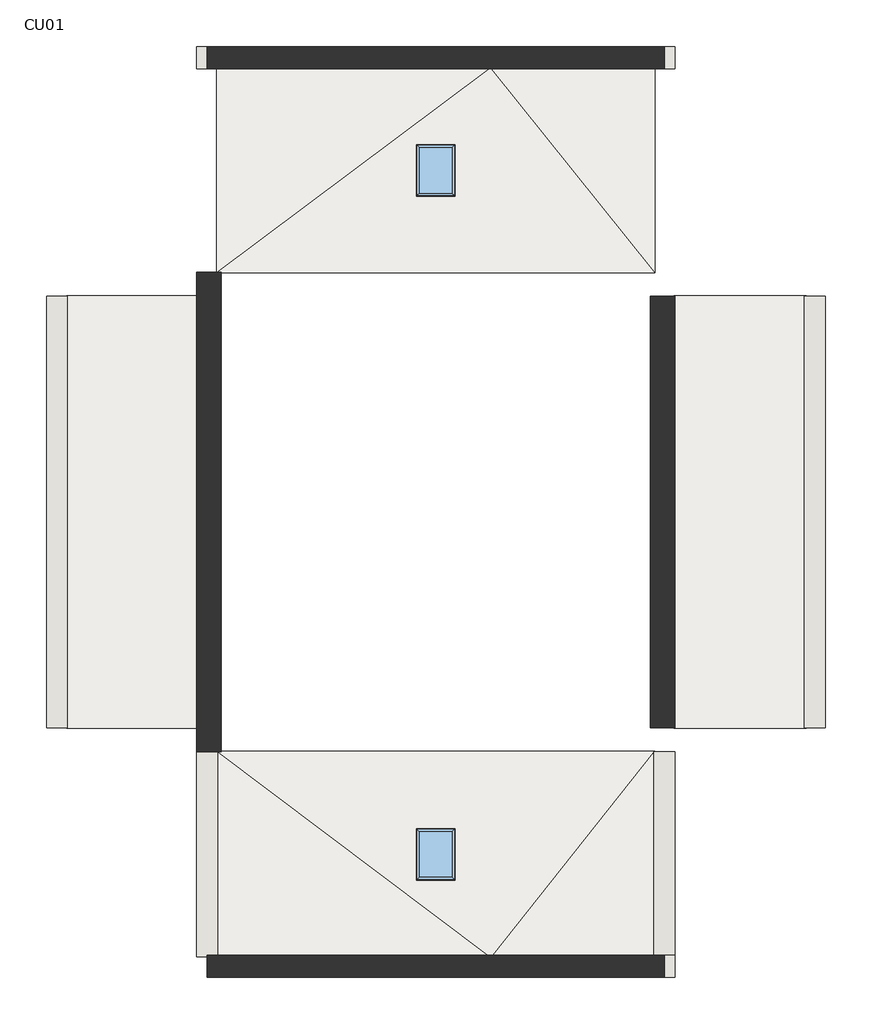
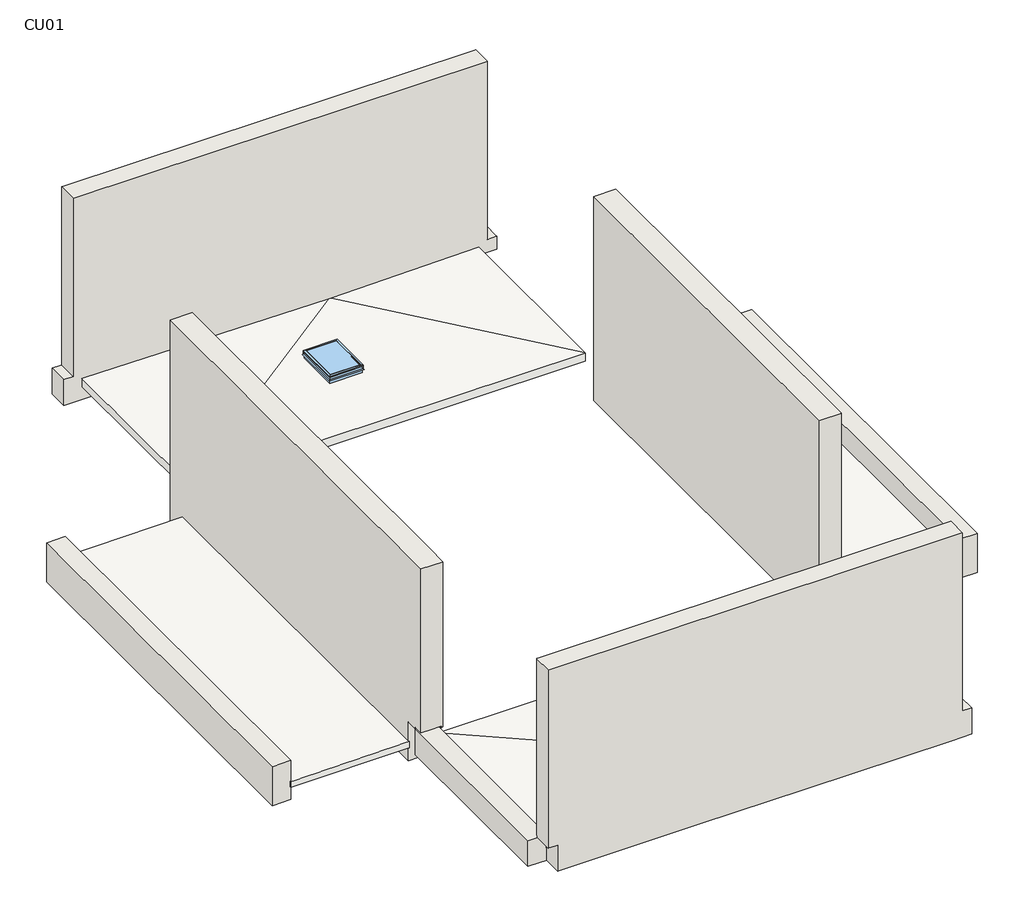
# One storey: 8 walls, 4 roofs, 2 windows.
"""IFC4 building model written with IfcOpenShell, lengths in millimetres."""

import ifcopenshell
import ifcopenshell.guid

model = None  # the IFC model being written
_history = None  # IfcOwnerHistory: only IFC2X3 demands one
_inside = {}  # id of a spatial element -> (the spatial element, [elements in it])
_under = {}  # id of a project, library or spatial element -> (it, [spatial elements below it])
_declared = {}  # id of a project -> (the project, [libraries it declares])
_typed = {}  # id of a type object -> (the type object, [elements of that type])
_made_of = {}  # id of a material, layer set ... -> (it, [elements and type objects made of it])


def new_model(schema):
    """Start an empty IFC model of exactly this schema.

    Asked for "IFC4X3", IfcOpenShell would pick the latest addendum, in which some entities
    have other attributes; the version numbers below select the first issue.
    IFC2X3 requires an IfcOwnerHistory on every rooted entity: one is made here for all.
    """
    global model, _history
    if schema == "IFC4X3":
        model = ifcopenshell.file(schema_version=(4, 3, 0, 0))
    else:
        model = ifcopenshell.file(schema=schema)
    _inside.clear()
    _under.clear()
    _declared.clear()
    _typed.clear()
    _made_of.clear()
    _history = None
    if model.schema == "IFC2X3":
        org = make("IfcOrganization", Name="unknown")
        user = make(
            "IfcPersonAndOrganization",
            ThePerson=make("IfcPerson", FamilyName="unknown"),
            TheOrganization=org,
        )
        app = make(
            "IfcApplication",
            ApplicationDeveloper=org,
            Version="unknown",
            ApplicationFullName="unknown",
            ApplicationIdentifier="unknown",
        )
        _history = make(
            "IfcOwnerHistory",
            OwningUser=user,
            OwningApplication=app,
            ChangeAction="ADDED",
            CreationDate=0,
        )
    return model


def make(cls, **values):
    """One entity of the class cls with the attributes given. An attribute that is None is left unset."""
    return model.create_entity(
        cls, **{name: value for name, value in values.items() if value is not None}
    )


def rooted(cls, **values):
    """An entity with a GlobalId (a new one), such as an element, a storey or a relation."""
    return make(cls, GlobalId=ifcopenshell.guid.new(), OwnerHistory=_history, **values)


def si_unit(unit_type, name, prefix=None):
    """IfcSIUnit, for example si_unit("LENGTHUNIT", "METRE", prefix="MILLI")."""
    return make("IfcSIUnit", UnitType=unit_type, Prefix=prefix, Name=name)


def assignment(units):
    """IfcUnitAssignment: the units of a project."""
    return None if units is None else make("IfcUnitAssignment", Units=units)


def point(xyz):
    """IfcCartesianPoint."""
    return None if xyz is None else make("IfcCartesianPoint", Coordinates=xyz)


def direction(xyz):
    """IfcDirection."""
    return None if xyz is None else make("IfcDirection", DirectionRatios=xyz)


def frame(location, z_axis=None, x_axis=None):
    """IfcAxis2Placement3D, a coordinate frame: its origin and axes. An axis left out is left unset."""
    return make(
        "IfcAxis2Placement3D",
        Location=point(location),
        Axis=direction(z_axis),
        RefDirection=direction(x_axis),
    )


def origin():
    """The frame at (0, 0, 0) with its axes left unset."""
    return frame((0.0, 0.0, 0.0))


def place(relative_to, where):
    """IfcLocalPlacement: puts the frame where relative to a parent placement (None: the world)."""
    return make(
        "IfcLocalPlacement", PlacementRelTo=relative_to, RelativePlacement=where
    )


def context(
    kind, dimensions, precision=None, world=None, true_north=None, identifier=None
):
    """IfcGeometricRepresentationContext, for example the 3D "Model" context."""
    return make(
        "IfcGeometricRepresentationContext",
        ContextIdentifier=identifier,
        ContextType=kind,
        CoordinateSpaceDimension=dimensions,
        Precision=precision,
        WorldCoordinateSystem=world,
        TrueNorth=true_north,
    )


def project(units=None, contexts=None):
    """IfcProject with its units and contexts."""
    return rooted(
        "IfcProject",
        Name="project",
        RepresentationContexts=contexts,
        UnitsInContext=assignment(units),
    )


def spatial(cls, under=None, at=None, **own):
    """A site, building, storey or space (cls), placed at a placement, below another one or the project."""
    s = rooted(cls, ObjectPlacement=at, **own)
    if under is not None:
        _under.setdefault(under.id(), (under, []))[1].append(s)
    return s


def polyline(points):
    """IfcPolyline through the points."""
    return make("IfcPolyline", Points=[point(p) for p in points])


def circle_curve(where, radius):
    """IfcCircle in the frame where."""
    return make("IfcCircle", Position=where, Radius=radius)


def outline(outer, holes=None, kind="AREA"):
    """IfcArbitraryClosedProfileDef: a profile drawn as a closed curve; with holes, ...WithVoids."""
    if holes is None:
        return make("IfcArbitraryClosedProfileDef", ProfileType=kind, OuterCurve=outer)
    return make(
        "IfcArbitraryProfileDefWithVoids",
        ProfileType=kind,
        OuterCurve=outer,
        InnerCurves=holes,
    )


def extrude(swept, where, along, depth):
    """IfcExtrudedAreaSolid: the profile swept, set in the frame where, extruded along a direction by depth."""
    return make(
        "IfcExtrudedAreaSolid",
        SweptArea=swept,
        Position=where,
        ExtrudedDirection=direction(along),
        Depth=depth,
    )


def faces_of(points, faces, orient=None, outer=None):
    """IfcFace entities. A face is a list of loops; a loop is a list of indices into points, from 0.

    orient and outer hold one flag for each loop. By default every Orientation is true, the
    first loop of a face is its IfcFaceOuterBound and the others are IfcFaceBound.
    """
    made = []
    for i, loops in enumerate(faces):
        bounds = []
        for j, loop in enumerate(loops):
            is_outer = j == 0 if outer is None else outer[i][j]
            bounds.append(
                make(
                    "IfcFaceOuterBound" if is_outer else "IfcFaceBound",
                    Bound=make("IfcPolyLoop", Polygon=[points[k] for k in loop]),
                    Orientation=True if orient is None else orient[i][j],
                )
            )
        made.append(make("IfcFace", Bounds=bounds))
    return made


def faceted_brep(points, faces, orient=None, outer=None, voids=None):
    """IfcFacetedBrep: a solid bounded by flat faces; with voids (closed shells), ...WithVoids."""
    shared = [point(p) for p in points]
    hull = make("IfcClosedShell", CfsFaces=faces_of(shared, faces, orient, outer))
    if voids is None:
        return make("IfcFacetedBrep", Outer=hull)
    return make(
        "IfcFacetedBrepWithVoids",
        Outer=hull,
        Voids=[
            make(cls, CfsFaces=faces_of(shared, fs, o, b)) for cls, fs, o, b in voids
        ],
    )


def shape(context_of_items, identifier, shape_type, items):
    """IfcShapeRepresentation: the items that make up one representation, for example the "Body"."""
    return make(
        "IfcShapeRepresentation",
        ContextOfItems=context_of_items,
        RepresentationIdentifier=identifier,
        RepresentationType=shape_type,
        Items=items,
    )


def source(mapping_origin, context_of_items, identifier, shape_type, items):
    """IfcRepresentationMap: a shape defined once, which mapped items show again and again."""
    return make(
        "IfcRepresentationMap",
        MappingOrigin=mapping_origin,
        MappedRepresentation=shape(context_of_items, identifier, shape_type, items),
    )


def transform(
    local_origin,
    x_axis=None,
    y_axis=None,
    z_axis=None,
    scale=None,
    scale2=None,
    scale3=None,
    uniform=True,
):
    """IfcCartesianTransformationOperator3D, or its non-uniform kind. x_axis, y_axis, z_axis: its Axis1, 2, 3."""
    if uniform:
        return make(
            "IfcCartesianTransformationOperator3D",
            Axis1=direction(x_axis),
            Axis2=direction(y_axis),
            LocalOrigin=point(local_origin),
            Scale=scale,
            Axis3=direction(z_axis),
        )
    return make(
        "IfcCartesianTransformationOperator3DnonUniform",
        Axis1=direction(x_axis),
        Axis2=direction(y_axis),
        LocalOrigin=point(local_origin),
        Scale=scale,
        Axis3=direction(z_axis),
        Scale2=scale2,
        Scale3=scale3,
    )


def mapped(mapping_source, mapping_target):
    """IfcMappedItem: shows the shape of a source again, moved by a transform."""
    return make(
        "IfcMappedItem", MappingSource=mapping_source, MappingTarget=mapping_target
    )


def made_of(thing, what):
    """Note that an element or type object is made of a material, layer set ...; save() writes the relation."""
    if what is not None:
        _made_of.setdefault(what.id(), (what, []))[1].append(thing)
    return thing


def element(
    cls,
    number,
    at=None,
    inside=None,
    cuts=None,
    type_object=None,
    material=None,
    context=None,
    identifier="Body",
    shape_type=None,
    held_by="IfcProductDefinitionShape",
    body=None,
    shapes=None,
    **own,
):
    """One element of the class cls, such as IfcWall. Its Tag is "e" and its number.

    at: its placement. inside: the storey or other place that contains it. cuts: it is an
    opening in that element (IfcRelVoidsElement). A single representation is given by context,
    identifier, shape_type and body (its items); several are given by shapes. held_by: the class
    of the entity that holds the representations. save() writes the other relations.
    """
    e = rooted(cls, Tag="e%d" % number, ObjectPlacement=at, **own)
    if body is not None:
        shapes = [shape(context, identifier, shape_type, body)]
    if shapes is not None:
        e.Representation = make(held_by, Representations=shapes)
    if inside is not None:
        _inside.setdefault(inside.id(), (inside, []))[1].append(e)
    if cuts is not None:
        rooted(
            "IfcRelVoidsElement", RelatingBuildingElement=cuts, RelatedOpeningElement=e
        )
    if type_object is not None:
        _typed.setdefault(type_object.id(), (type_object, []))[1].append(e)
    return made_of(e, material)


def aggregate(whole, parts):
    """IfcRelAggregates: a whole, such as a stair, and the parts it consists of."""
    return rooted("IfcRelAggregates", RelatingObject=whole, RelatedObjects=parts)


def save(model, path):
    """Write the relations noted so far, then the file.

    IfcRelAggregates (storeys below a building ...), IfcRelContainedInSpatialStructure (elements
    in a storey), IfcRelDefinesByType, IfcRelAssociatesMaterial and IfcRelDeclares: one each for
    every whole, place, type object, material and project.
    """
    for whole, parts in _under.values():
        aggregate(whole, parts)
    for where, things in _inside.values():
        rooted(
            "IfcRelContainedInSpatialStructure",
            RelatedElements=things,
            RelatingStructure=where,
        )
    for kind, things in _typed.values():
        rooted("IfcRelDefinesByType", RelatedObjects=things, RelatingType=kind)
    for what, things in _made_of.values():
        rooted("IfcRelAssociatesMaterial", RelatedObjects=things, RelatingMaterial=what)
    for by, libraries in _declared.values():
        rooted("IfcRelDeclares", RelatingContext=by, RelatedDefinitions=libraries)
    model.write(path)


def plane_surface(at):
    """IfcPlane: the flat surface through the origin of the frame at, square to its z axis."""
    return make("IfcPlane", Position=at)


def cylinder_surface(at, radius):
    """IfcCylindricalSurface: all points at the distance radius from the z axis of the frame at."""
    return make("IfcCylindricalSurface", Position=at, Radius=radius)


def advanced_brep(points, edges, surfaces, faces):
    """IfcAdvancedBrep: a solid bounded by faces that lie on surfaces and meet in shared edges.

    An edge is (start, end): straight between two places in points (the first is 0);
    or (start, end, curve); or (start, end, curve, False) where it runs against its curve.
    A face is (place in surfaces, loops), or (place, loops, False) where it looks against
    its surface's normal. A loop lists edges by number (the first is 1), with a minus sign
    where the edge is run from its end to its start. The first loop is the outer one.
    """
    corners = [point(p) for p in points]
    vertices = [make("IfcVertexPoint", VertexGeometry=c) for c in corners]
    made = []
    for start, end, *more in edges:
        made.append(
            make(
                "IfcEdgeCurve",
                EdgeStart=vertices[start],
                EdgeEnd=vertices[end],
                EdgeGeometry=more[0] if more else make("IfcPolyline", Points=[corners[start], corners[end]]),
                SameSense=more[1] if len(more) > 1 else True,
            )
        )
    hull = []
    for where, loops, *sense in faces:
        bounds = []
        for j, loop in enumerate(loops):
            ring = [make("IfcOrientedEdge", EdgeElement=made[abs(k) - 1], Orientation=k > 0) for k in loop]
            bounds.append(
                make(
                    "IfcFaceOuterBound" if j == 0 else "IfcFaceBound",
                    Bound=make("IfcEdgeLoop", EdgeList=ring),
                    Orientation=True,
                )
            )
        hull.append(make("IfcAdvancedFace", Bounds=bounds, FaceSurface=surfaces[where], SameSense=sense[0] if sense else True))
    return make("IfcAdvancedBrep", Outer=make("IfcClosedShell", CfsFaces=hull))


def claraboya_0711_x_0965mm_26b2130f(model_context):
    return source(origin(), model_context, "Body", "SolidModel", [
        faceted_brep([(254.440073, 370.1040988, 4001.2), (279.840073, 395.5040988, 4001.2), (279.840073, -569.4959012, 4001.2), (254.440073, -544.0959012, 4001.2), (254.440073, 370.1040988, 4026.6), (254.440073, -544.0959012, 4026.6), (292.540073, 408.2040988, 4026.6), (292.540073, -582.1959012, 4026.6), (292.540073, 408.2040988, 4001.2), (292.540073, -582.1959012, 4001.2), (292.540073, 408.2040988, 3950.4), (292.540073, -582.1959012, 3950.4), (307.1089145, 422.7729403, 3929.5935381), (307.1089145, -596.7647427, 3929.5935381), (301.907299, 417.5713248, 3925.9513277), (301.907299, -591.5631272, 3925.9513277), (286.190073, 401.8540988, 3948.3978527), (286.190073, -575.8459012, 3948.3978527), (286.190073, 401.8540988, 4001.2), (286.190073, -575.8459012, 4001.2), (-431.159927, -569.4959012, 4001.2), (-405.759927, -544.0959012, 4001.2), (-405.759927, -544.0959012, 4026.6), (-443.859927, -582.1959012, 4026.6), (-443.859927, -582.1959012, 4001.2), (-443.859927, -582.1959012, 3950.4), (-458.4287685, -596.7647427, 3929.5935381), (-453.227153, -591.5631272, 3925.9513277), (-437.509927, -575.8459012, 3948.3978527), (-437.509927, -575.8459012, 4001.2), (-431.159927, 395.5040988, 4001.2), (-405.759927, 370.1040988, 4001.2), (-405.759927, 370.1040988, 4026.6), (-443.859927, 408.2040988, 4026.6), (-443.859927, 408.2040988, 4001.2), (-443.859927, 408.2040988, 3950.4), (-458.4287685, 422.7729403, 3929.5935381), (-453.227153, 417.5713248, 3925.9513277), (-437.509927, 401.8540988, 3948.3978527), (-437.509927, 401.8540988, 4001.2)], [[[0, 1, 2, 3]], [[4, 0, 3, 5]], [[6, 4, 5, 7]], [[8, 6, 7, 9]], [[10, 8, 9, 11]], [[12, 10, 11, 13]], [[14, 12, 13, 15]], [[16, 14, 15, 17]], [[18, 16, 17, 19]], [[1, 18, 19, 2]], [[3, 2, 20, 21]], [[5, 3, 21, 22]], [[7, 5, 22, 23]], [[9, 7, 23, 24]], [[11, 9, 24, 25]], [[13, 11, 25, 26]], [[15, 13, 26, 27]], [[17, 15, 27, 28]], [[19, 17, 28, 29]], [[2, 19, 29, 20]], [[21, 20, 30, 31]], [[22, 21, 31, 32]], [[23, 22, 32, 33]], [[24, 23, 33, 34]], [[25, 24, 34, 35]], [[26, 25, 35, 36]], [[27, 26, 36, 37]], [[28, 27, 37, 38]], [[29, 28, 38, 39]], [[20, 29, 39, 30]], [[31, 30, 1, 0]], [[32, 31, 0, 4]], [[33, 32, 4, 6]], [[34, 33, 6, 8]], [[35, 34, 8, 10]], [[36, 35, 10, 12]], [[37, 36, 12, 14]], [[38, 37, 14, 16]], [[39, 38, 16, 18]], [[30, 39, 18, 1]]]),
        faceted_brep([(279.840073, -569.4959012, 4001.2), (279.840073, -569.4959012, 3848.8), (279.840073, 395.5040988, 3848.8), (279.840073, 395.5040988, 4001.2), (254.440073, -544.0959012, 4001.2), (254.440073, 370.1040988, 4001.2), (254.440073, -544.0959012, 3975.8), (254.440073, 370.1040988, 3975.8), (235.390073, -525.0459012, 3975.8), (235.390073, 351.0540988, 3975.8), (235.390073, -525.0459012, 3848.8), (235.390073, 351.0540988, 3848.8), (-431.159927, 395.5040988, 3848.8), (-431.159927, 395.5040988, 4001.2), (-405.759927, 370.1040988, 4001.2), (-405.759927, 370.1040988, 3975.8), (-386.709927, 351.0540988, 3975.8), (-386.709927, 351.0540988, 3848.8), (-431.159927, -569.4959012, 3848.8), (-431.159927, -569.4959012, 4001.2), (-405.759927, -544.0959012, 4001.2), (-405.759927, -544.0959012, 3975.8), (-386.709927, -525.0459012, 3975.8), (-386.709927, -525.0459012, 3848.8)], [[[0, 1, 2, 3]], [[4, 0, 3, 5]], [[6, 4, 5, 7]], [[8, 6, 7, 9]], [[10, 8, 9, 11]], [[1, 10, 11, 2]], [[3, 2, 12, 13]], [[5, 3, 13, 14]], [[7, 5, 14, 15]], [[9, 7, 15, 16]], [[11, 9, 16, 17]], [[2, 11, 17, 12]], [[13, 12, 18, 19]], [[14, 13, 19, 20]], [[15, 14, 20, 21]], [[16, 15, 21, 22]], [[17, 16, 22, 23]], [[12, 17, 23, 18]], [[19, 18, 1, 0]], [[20, 19, 0, 4]], [[21, 20, 4, 6]], [[22, 21, 6, 8]], [[23, 22, 8, 10]], [[18, 23, 10, 1]]]),
        extrude(outline(polyline([(254.440073, -544.0959012), (-405.759927, -544.0959012), (-405.759927, 370.1040988), (254.440073, 370.1040988), (254.440073, -544.0959012)])), frame((0.0, 0.0, 4020.25), z_axis=(0.0, 0.0, 1.0), x_axis=(1.0, 0.0, 0.0)), (0.0, 0.0, 1.0), 6.35),
    ])


def claraboya_0711_x_0965mm_17ef4467(model_context):
    return source(origin(), model_context, "Body", "SolidModel", [
        faceted_brep([(254.440073, -370.1040988, 4001.2), (254.440073, 544.0959012, 4001.2), (279.840073, 569.4959012, 4001.2), (279.840073, -395.5040988, 4001.2), (254.440073, -370.1040988, 4026.6), (254.440073, 544.0959012, 4026.6), (292.540073, -408.2040988, 4026.6), (292.540073, 582.1959012, 4026.6), (292.540073, -408.2040988, 4001.2), (292.540073, 582.1959012, 4001.2), (292.540073, -408.2040988, 3950.4), (292.540073, 582.1959012, 3950.4), (307.1089145, -422.7729403, 3929.5935381), (307.1089145, 596.7647427, 3929.5935381), (301.907299, -417.5713248, 3925.9513277), (301.907299, 591.5631272, 3925.9513277), (286.190073, -401.8540988, 3948.3978527), (286.190073, 575.8459012, 3948.3978527), (286.190073, -401.8540988, 4001.2), (286.190073, 575.8459012, 4001.2), (-405.759927, 544.0959012, 4001.2), (-431.159927, 569.4959012, 4001.2), (-405.759927, 544.0959012, 4026.6), (-443.859927, 582.1959012, 4026.6), (-443.859927, 582.1959012, 4001.2), (-443.859927, 582.1959012, 3950.4), (-458.4287685, 596.7647427, 3929.5935381), (-453.227153, 591.5631272, 3925.9513277), (-437.509927, 575.8459012, 3948.3978527), (-437.509927, 575.8459012, 4001.2), (-405.759927, -370.1040988, 4001.2), (-431.159927, -395.5040988, 4001.2), (-405.759927, -370.1040988, 4026.6), (-443.859927, -408.2040988, 4026.6), (-443.859927, -408.2040988, 4001.2), (-443.859927, -408.2040988, 3950.4), (-458.4287685, -422.7729403, 3929.5935381), (-453.227153, -417.5713248, 3925.9513277), (-437.509927, -401.8540988, 3948.3978527), (-437.509927, -401.8540988, 4001.2)], [[[0, 1, 2, 3]], [[4, 5, 1, 0]], [[6, 7, 5, 4]], [[8, 9, 7, 6]], [[10, 11, 9, 8]], [[12, 13, 11, 10]], [[14, 15, 13, 12]], [[16, 17, 15, 14]], [[18, 19, 17, 16]], [[3, 2, 19, 18]], [[1, 20, 21, 2]], [[5, 22, 20, 1]], [[7, 23, 22, 5]], [[9, 24, 23, 7]], [[11, 25, 24, 9]], [[13, 26, 25, 11]], [[15, 27, 26, 13]], [[17, 28, 27, 15]], [[19, 29, 28, 17]], [[2, 21, 29, 19]], [[20, 30, 31, 21]], [[22, 32, 30, 20]], [[23, 33, 32, 22]], [[24, 34, 33, 23]], [[25, 35, 34, 24]], [[26, 36, 35, 25]], [[27, 37, 36, 26]], [[28, 38, 37, 27]], [[29, 39, 38, 28]], [[21, 31, 39, 29]], [[30, 0, 3, 31]], [[32, 4, 0, 30]], [[33, 6, 4, 32]], [[34, 8, 6, 33]], [[35, 10, 8, 34]], [[36, 12, 10, 35]], [[37, 14, 12, 36]], [[38, 16, 14, 37]], [[39, 18, 16, 38]], [[31, 3, 18, 39]]]),
        faceted_brep([(279.840073, 569.4959012, 4001.2), (279.840073, -395.5040988, 4001.2), (279.840073, -395.5040988, 3848.8), (279.840073, 569.4959012, 3848.8), (254.440073, 544.0959012, 4001.2), (254.440073, -370.1040988, 4001.2), (254.440073, 544.0959012, 3975.8), (254.440073, -370.1040988, 3975.8), (235.390073, 525.0459012, 3975.8), (235.390073, -351.0540988, 3975.8), (235.390073, 525.0459012, 3848.8), (235.390073, -351.0540988, 3848.8), (-431.159927, -395.5040988, 4001.2), (-431.159927, -395.5040988, 3848.8), (-405.759927, -370.1040988, 4001.2), (-405.759927, -370.1040988, 3975.8), (-386.709927, -351.0540988, 3975.8), (-386.709927, -351.0540988, 3848.8), (-431.159927, 569.4959012, 4001.2), (-431.159927, 569.4959012, 3848.8), (-405.759927, 544.0959012, 4001.2), (-405.759927, 544.0959012, 3975.8), (-386.709927, 525.0459012, 3975.8), (-386.709927, 525.0459012, 3848.8)], [[[0, 1, 2, 3]], [[4, 5, 1, 0]], [[6, 7, 5, 4]], [[8, 9, 7, 6]], [[10, 11, 9, 8]], [[3, 2, 11, 10]], [[1, 12, 13, 2]], [[5, 14, 12, 1]], [[7, 15, 14, 5]], [[9, 16, 15, 7]], [[11, 17, 16, 9]], [[2, 13, 17, 11]], [[12, 18, 19, 13]], [[14, 20, 18, 12]], [[15, 21, 20, 14]], [[16, 22, 21, 15]], [[17, 23, 22, 16]], [[13, 19, 23, 17]], [[18, 0, 3, 19]], [[20, 4, 0, 18]], [[21, 6, 4, 20]], [[22, 8, 6, 21]], [[23, 10, 8, 22]], [[19, 3, 10, 23]]]),
        extrude(outline(polyline([(254.440073, 544.0959012), (254.440073, -370.1040988), (-405.759927, -370.1040988), (-405.759927, 544.0959012), (254.440073, 544.0959012)])), frame((0.0, 0.0, 4020.25), z_axis=(0.0, 0.0, 1.0), x_axis=(1.0, 0.0, 0.0)), (0.0, 0.0, 1.0), 6.35),
    ])


model = new_model("IFC4")

# Units and contexts
model_context = context("Model", 3, world=origin())
ifc_project = project(units=[si_unit("LENGTHUNIT", "METRE", prefix="MILLI")], contexts=[model_context])

# Site, building, storey
site = spatial("IfcSite", under=ifc_project)
building = spatial("IfcBuilding", under=site)
storey = spatial("IfcBuildingStorey", under=building, Name="CU01", Elevation=2430.0)

# Roofs
placement = place(None, origin())
element("IfcRoof", 1, ObjectType="ACAB CUB GRAVA INF-A_PABLO", at=placement, inside=storey, context=model_context, shape_type="Brep", body=[
    faceted_brep([(-12165.0, -4267.5, 2730.0), (-12165.0, -4252.5, 2730.0), (-12165.0, -232.5, 2730.0), (-12165.0, -217.5, 2730.0), (-12165.0, -217.5, 2921.2), (-12165.0, -232.5, 2921.2), (-12165.0, -4252.5, 2921.2), (-12165.0, -4267.5, 2921.2), (-12235.0, -217.5, 2730.0), (-20835.0, -217.5, 2730.0), (-20835.0, -217.5, 2921.2), (-15415.0, -217.5, 2871.2), (-16188.95, -1804.45, 2890.7919753), (-16188.95, -1804.45, 2730.0), (-16188.95, -2680.55, 2730.0), (-16188.95, -2680.55, 2901.6080247), (-16811.05, -2680.55, 2730.0), (-16811.05, -2680.55, 2901.6080247), (-16811.05, -1804.45, 2730.0), (-16811.05, -1804.45, 2890.7919753), (-20750.0, -4267.5, 2730.0), (-20835.0, -4267.5, 2730.0), (-20835.0, -4252.5, 2730.0), (-20835.0, -232.5, 2730.0), (-20835.0, -4267.5, 2921.2), (-20835.0, -4252.5, 2921.2), (-20835.0, -232.5, 2921.2), (-20750.0, -4267.5, 2921.2), (-12177.037037, -4252.5, 2921.0148148), (-12180.0, -4248.8076923, 2920.9692308), (-15402.962963, -232.5, 2871.3851852), (-15435.0740741, -232.5, 2871.3851852)], [[[0, 1, 2, 3, 4, 5, 6, 7]], [[3, 8, 9, 10, 11, 4]], [[12, 13, 14, 15]], [[15, 14, 16, 17]], [[17, 16, 18, 19]], [[13, 12, 19, 18]], [[3, 2, 1, 0, 20, 21, 22, 23, 9, 8], [14, 13, 18, 16]], [[9, 23, 22, 21, 24, 25, 26, 10]], [[0, 7, 27, 24, 21, 20]], [[24, 27, 7, 28, 29, 30, 11, 31], [12, 15, 17, 19]], [[7, 6, 5, 4, 11, 30, 29, 28]], [[10, 26, 25, 24, 31, 11]]]),
])
element("IfcRoof", 2, ObjectType="ACAB CUB GRAVA INF-B_PABLO", at=placement, inside=storey, context=model_context, shape_type="Brep", body=[
    faceted_brep([(-23810.0, -4717.5, 2430.0), (-21230.0, -4717.5, 2430.0), (-21215.0, -4717.5, 2430.0), (-21215.0, -13267.5, 2430.0), (-21215.0, -13282.5, 2430.0), (-21230.0, -13282.5, 2430.0), (-23810.0, -13282.5, 2430.0), (-23810.0, -13267.5, 2430.0), (-23810.0, -4732.5, 2430.0), (-21215.0, -4717.5, 2581.2), (-23810.0, -4717.5, 2551.2), (-21230.0, -4717.5, 2581.0265896), (-23810.0, -13282.5, 2551.2), (-23810.0, -13267.5, 2551.2), (-23810.0, -9000.0, 2551.2), (-23810.0, -4732.5, 2551.2), (-21215.0, -13282.5, 2581.2), (-21215.0, -13267.5, 2581.2)], [[[0, 1, 2, 3, 4, 5, 6, 7, 8]], [[9, 2, 1, 0, 10, 11]], [[10, 0, 8, 7, 6, 12, 13, 14, 15]], [[12, 6, 5, 4, 16]], [[10, 15, 14, 13, 12, 16, 17, 9, 11]], [[16, 4, 3, 2, 9, 17]]]),
])
element("IfcRoof", 3, ObjectType="ACAB CUB GRAVA INF-A_PABLO", at=placement, inside=storey, context=model_context, shape_type="Brep", body=[
    faceted_brep([(-12165.0, -17812.5, 2730.0), (-12165.0, -17767.5, 2730.0), (-12165.0, -13747.5, 2730.0), (-12165.0, -13732.5, 2730.0), (-12165.0, -13732.5, 2921.2), (-12165.0, -13747.5, 2921.2), (-12165.0, -17767.5, 2921.2), (-12165.0, -17812.5, 2921.2), (-15405.0, -17812.5, 2871.2), (-20820.0, -17812.5, 2921.0618785), (-20835.0, -17812.5, 2921.2), (-20835.0, -17812.5, 2730.0), (-20820.0, -17812.5, 2730.0), (-16188.95, -16210.55, 2730.0), (-16188.95, -16210.55, 2890.8317402), (-16188.95, -15334.45, 2901.5682598), (-16188.95, -15334.45, 2730.0), (-16811.05, -15334.45, 2901.5682598), (-16811.05, -15334.45, 2730.0), (-16811.05, -16210.55, 2890.8317402), (-16811.05, -16210.55, 2730.0), (-20835.0, -17797.5, 2730.0), (-20835.0, -13732.5, 2730.0), (-20820.0, -13732.5, 2730.0), (-20750.0, -13732.5, 2730.0), (-20835.0, -17797.5, 2921.2), (-20835.0, -13732.5, 2921.2), (-20820.0, -13732.5, 2921.2), (-20750.0, -13732.5, 2921.2), (-12176.9117647, -13747.5, 2921.0161765), (-12180.0, -13751.3888889, 2920.9685185), (-15369.2647059, -17767.5, 2871.7514706), (-20820.0, -13743.7707182, 2921.0618785), (-15464.8897059, -17767.5, 2871.7514706)], [[[0, 1, 2, 3, 4, 5, 6, 7]], [[0, 7, 8, 9, 10, 11, 12]], [[13, 14, 15, 16]], [[16, 15, 17, 18]], [[18, 17, 19, 20]], [[14, 13, 20, 19]], [[3, 2, 1, 0, 12, 11, 21, 22, 23, 24], [13, 16, 18, 20]], [[22, 21, 11, 10, 25, 26]], [[4, 3, 24, 23, 22, 26, 27, 28]], [[7, 6, 5, 4, 29, 30, 31, 8]], [[4, 28, 27, 26, 32, 33, 8, 31, 30, 29], [15, 14, 19, 17]], [[26, 25, 10, 9, 8, 33, 32]]]),
])
element("IfcRoof", 4, ObjectType="ACAB CUB GRAVA INF-B_PABLO", at=placement, inside=storey, context=model_context, shape_type="Brep", body=[
    faceted_brep([(-11785.0, -4717.5, 2430.0), (-9165.0, -4717.5, 2430.0), (-9165.0, -4732.5, 2430.0), (-9165.0, -13267.5, 2430.0), (-9165.0, -13282.5, 2430.0), (-11785.0, -13282.5, 2430.0), (-11785.0, -13267.5, 2430.0), (-11785.0, -4732.5, 2430.0), (-9165.0, -4717.5, 2551.2), (-11785.0, -4717.5, 2581.2), (-9165.0, -13282.5, 2551.2), (-9165.0, -4732.5, 2551.2), (-9165.0, -9000.0, 2551.2), (-9165.0, -13267.5, 2551.2), (-11785.0, -13282.5, 2581.2), (-11785.0, -4732.5, 2581.2), (-11785.0, -13267.5, 2581.2)], [[[0, 1, 2, 3, 4, 5, 6, 7]], [[8, 1, 0, 9]], [[10, 4, 3, 2, 1, 8, 11, 12, 13]], [[14, 5, 4, 10]], [[12, 11, 8, 9, 15, 16, 14, 10, 13]], [[9, 0, 7, 6, 5, 14, 16, 15]]]),
])

# Walls
element("IfcWall", 5, ObjectType="MURO TIPO 1_EXTERIOR_PETO_PABLO", at=placement, inside=storey, context=model_context, shape_type="Brep", body=[
    faceted_brep([(-23795.0, -13267.5, 2130.0), (-23795.0, -4732.5, 2130.0), (-23795.0, -4732.5, 2430.0), (-23795.0, -13267.5, 2430.0), (-23795.0, -4732.5, 3030.0), (-23795.0, -13267.5, 3030.0), (-23795.0, -13267.5, 2551.3734104), (-23795.0, -4732.5, 2551.3734104), (-24205.0, -4732.5, 2130.0), (-24205.0, -13267.5, 2130.0), (-24205.0, -13267.5, 3030.0), (-24205.0, -4732.5, 3030.0), (-23810.0, -13267.5, 2430.0), (-23810.0, -13267.5, 2551.2), (-23810.0, -4732.5, 2551.2), (-23810.0, -4732.5, 2430.0), (-23810.0, -9000.0, 2551.2)], [[[0, 1, 2, 3]], [[4, 5, 6, 7]], [[8, 9, 10, 11]], [[1, 0, 9, 8]], [[5, 4, 11, 10]], [[5, 10, 9, 0, 3, 12, 13, 6]], [[1, 8, 11, 4, 7, 14, 15, 2]], [[15, 12, 3, 2]], [[12, 15, 14, 16, 13]], [[13, 16, 14, 7, 6]]]),
])
element("IfcWall", 6, ObjectType="MURO TIPO 1_EXTERIOR_PETO_PABLO", at=placement, inside=storey, context=model_context, shape_type="Brep", body=[
    faceted_brep([(-8795.0, -13267.5, 2130.0), (-8795.0, -4732.5, 2130.0), (-8795.0, -4732.5, 3030.0), (-8795.0, -13267.5, 3030.0), (-9205.0, -4732.5, 2130.0), (-9205.0, -13267.5, 2130.0), (-9205.0, -13267.5, 2430.0), (-9205.0, -4732.5, 2430.0), (-9205.0, -13267.5, 3030.0), (-9205.0, -4732.5, 3030.0), (-9205.0, -4732.5, 2551.6580153), (-9205.0, -13267.5, 2551.6580153), (-9165.0, -13267.5, 2551.2), (-9165.0, -13267.5, 2430.0), (-9165.0, -4732.5, 2430.0), (-9165.0, -4732.5, 2551.2), (-9165.0, -9000.0, 2551.2)], [[[0, 1, 2, 3]], [[4, 5, 6, 7]], [[8, 9, 10, 11]], [[1, 0, 5, 4]], [[3, 2, 9, 8]], [[0, 3, 8, 11, 12, 13, 6, 5]], [[2, 1, 4, 7, 14, 15, 10, 9]], [[13, 14, 7, 6]], [[14, 13, 12, 16, 15]], [[16, 12, 11, 10, 15]]]),
])
element("IfcWall", 7, ObjectType="MURO TIPO 1_EXTERIOR_PETO-CUB_PABLO", at=placement, inside=storey, context=model_context, shape_type="Brep", body=[
    faceted_brep([(-21230.0, -232.5, 2430.0), (-12235.0, -232.5, 2430.0), (-12235.0, -232.5, 2730.0), (-20835.0, -232.5, 2730.0), (-20835.0, -232.5, 2921.2), (-15435.0740741, -232.5, 2871.3851852), (-15402.962963, -232.5, 2871.3851852), (-12180.0, -232.5, 2920.9692308), (-12165.0, -232.5, 2921.2), (-12165.0, -232.5, 2730.0), (-11770.0, -232.5, 2730.0), (-11770.0, -232.5, 3030.0), (-11975.0, -232.5, 3030.0), (-11975.0, -232.5, 7150.0), (-12002.5, -232.5, 7150.0), (-21010.0, -232.5, 7150.0), (-21025.0, -232.5, 7150.0), (-21025.0, -232.5, 3030.0), (-21230.0, -232.5, 3030.0), (-21230.0, -232.5, 2730.0), (-12235.0, 207.5, 2430.0), (-17710.0, 207.5, 2430.0), (-21230.0, 207.5, 2430.0), (-21230.0, 207.5, 3030.0), (-21025.0, 207.5, 3030.0), (-21025.0, 207.5, 7150.0), (-21010.0, 207.5, 7150.0), (-12002.5, 207.5, 7150.0), (-11975.0, 207.5, 7150.0), (-11975.0, 207.5, 3030.0), (-11770.0, 207.5, 3030.0), (-11770.0, 207.5, 2730.0), (-12235.0, 207.5, 2730.0), (-12165.0, -217.5, 2730.0), (-12235.0, -217.5, 2730.0), (-12165.0, -217.5, 2921.2), (-15415.0, -217.5, 2871.2), (-20835.0, -217.5, 2921.2), (-20835.0, -217.5, 2730.0), (-21230.0, 192.5, 3030.0), (-21230.0, -217.5, 3030.0), (-11770.0, -217.5, 3030.0), (-11770.0, 192.5, 3030.0)], [[[0, 1, 2, 3, 4, 5, 6, 7, 8, 9, 10, 11, 12, 13, 14, 15, 16, 17, 18, 19]], [[20, 21, 22, 23, 24, 25, 26, 27, 28, 29, 30, 31, 32]], [[1, 0, 22, 21, 20]], [[16, 15, 14, 13, 28, 27, 26, 25]], [[32, 31, 10, 9, 33, 34]], [[2, 1, 20, 32, 34]], [[33, 35, 36, 37, 38, 34]], [[35, 33, 9, 8]], [[34, 38, 3, 2]], [[38, 37, 4, 3]], [[16, 25, 24, 17]], [[17, 24, 23, 39, 40, 18]], [[22, 0, 19, 18, 40, 39, 23]], [[36, 35, 8, 7, 6]], [[37, 36, 5, 4]], [[36, 6, 5]], [[28, 13, 12, 29]], [[29, 12, 11, 41, 42, 30]], [[11, 10, 31, 30, 42, 41]]]),
])
element("IfcWall", 8, ObjectType="MURO TIPO 3B_ESTAR-EXT_YESO-CEMENTO_PABLO", at=placement, inside=storey, context=model_context, shape_type="Brep", body=[
    faceted_brep([(-12250.0, -4732.5, 2130.0), (-12250.0, -13267.5, 2130.0), (-12250.0, -13267.5, 6850.0), (-12250.0, -4732.5, 6850.0), (-11770.0, -13267.5, 2130.0), (-11770.0, -4732.5, 2130.0), (-11770.0, -4732.5, 2430.0), (-11770.0, -13267.5, 2430.0), (-11770.0, -4732.5, 6850.0), (-11770.0, -13267.5, 6850.0), (-11770.0, -13267.5, 2581.0282443), (-11770.0, -4732.5, 2581.0282443), (-11785.0, -13267.5, 2130.0), (-11785.0, -13267.5, 6850.0), (-11785.0, -4732.5, 2430.0), (-11785.0, -13267.5, 2430.0), (-11785.0, -13267.5, 2581.2), (-11785.0, -4732.5, 2581.2)], [[[0, 1, 2, 3]], [[4, 5, 6, 7]], [[8, 9, 10, 11]], [[1, 0, 5, 4, 12]], [[3, 2, 13, 9, 8]], [[14, 15, 7, 6]], [[16, 17, 11, 10]], [[15, 14, 17, 16]], [[1, 12, 4, 7, 15, 16, 10, 9, 13, 2]], [[5, 0, 3, 8, 11, 17, 14, 6]]]),
])
element("IfcWall", 9, ObjectType="MURO TIPO 1_EXTERIOR_PETO_PABLO", at=placement, inside=storey, context=model_context, shape_type="Brep", body=[
    faceted_brep([(-11770.0, -17767.5, 2430.0), (-11770.0, -13747.5, 2430.0), (-11770.0, -13747.5, 3030.0), (-11770.0, -17767.5, 3030.0), (-12180.0, -13747.5, 2430.0), (-12180.0, -17767.5, 2430.0), (-12180.0, -17767.5, 2730.0), (-12180.0, -13747.5, 2730.0), (-12180.0, -17767.5, 3030.0), (-12180.0, -13747.5, 3030.0), (-12180.0, -13747.5, 2921.0161765), (-12180.0, -13751.3888889, 2920.9685185), (-12180.0, -17767.5, 2920.9685185), (-11975.0, -17767.5, 3030.0), (-12165.0, -13747.5, 2921.2), (-12165.0, -13747.5, 2730.0), (-12165.0, -17767.5, 2730.0), (-12165.0, -17767.5, 2921.2), (-12176.9117647, -13747.5, 2921.0161765)], [[[0, 1, 2, 3]], [[4, 5, 6, 7]], [[8, 9, 10, 11, 12]], [[1, 0, 5, 4]], [[3, 2, 9, 8, 13]], [[14, 15, 16, 17]], [[7, 6, 16, 15]], [[11, 18, 14, 17, 12]], [[18, 11, 10]], [[2, 1, 4, 7, 15, 14, 18, 10, 9]], [[0, 3, 13, 8, 12, 17, 16, 6, 5]]]),
])
element("IfcWall", 10, ObjectType="MURO TIPO 1_EXTERIOR_PETO_PABLO", at=placement, inside=storey, context=model_context, shape_type="Brep", body=[
    faceted_brep([(-20820.0, -17797.5, 2430.0), (-20820.0, -17767.5, 2430.0), (-20820.0, -13537.5, 2430.0), (-20820.0, -13537.5, 3030.0), (-20820.0, -17767.5, 3030.0), (-20820.0, -17797.5, 3030.0), (-20820.0, -17797.5, 2921.0618785), (-20820.0, -17767.5, 2921.0618785), (-20820.0, -13743.7707182, 2921.0618785), (-20820.0, -13732.5, 2921.2), (-20820.0, -13732.5, 2730.0), (-20820.0, -17767.5, 2730.0), (-20820.0, -17797.5, 2730.0), (-21230.0, -13537.5, 2430.0), (-21230.0, -17797.5, 2430.0), (-21230.0, -17797.5, 3030.0), (-21230.0, -13537.5, 3030.0), (-21010.0, -17797.5, 3030.0), (-20835.0, -13732.5, 2730.0), (-20835.0, -17797.5, 2730.0), (-20835.0, -13732.5, 2921.2), (-20835.0, -17797.5, 2921.2)], [[[0, 1, 2, 3, 4, 5, 6, 7, 8, 9, 10, 11, 12]], [[13, 14, 15, 16]], [[2, 1, 0, 14, 13]], [[5, 4, 3, 16, 15, 17]], [[10, 18, 19, 12, 11]], [[18, 20, 21, 19]], [[20, 9, 8]], [[20, 8, 7, 6, 21]], [[3, 2, 13, 16]], [[20, 18, 10, 9]], [[5, 17, 15, 14, 0, 12, 19, 21, 6]]]),
])
element("IfcWall", 11, ObjectType="MURO TIPO 3B_ESTAR-EXT_YESO-CEMENTO_PABLO", at=placement, inside=storey, context=model_context, shape_type="AdvancedBrep", body=[
    advanced_brep(
    [(-21230.0, -4252.5, 2130.0), (-21230.0, -13267.5, 2130.0), (-21230.0, -13267.5, 2430.0), (-21230.0, -13267.5, 3030.0), (-21230.0, -13537.5, 3030.0), (-21230.0, -13537.5, 3060.7854779), (-21230.0, -13747.5, 3060.7854779), (-21230.0, -13747.5, 6850.0), (-21230.0, -4252.5, 6850.0), (-20750.0, -13267.5, 2130.0), (-20750.0, -4732.5, 2130.0), (-20750.0, -4252.5, 2130.0), (-20750.0, -4252.5, 2730.0), (-20750.0, -4252.5, 2921.0148148), (-20750.0, -4252.5, 6850.0), (-20750.0, -4732.5, 6850.0), (-20750.0, -13267.5, 6850.0), (-20750.0, -13747.5, 6850.0), (-20750.0, -13747.5, 3030.0), (-20750.0, -13537.5, 3030.0), (-20750.0, -13267.5, 3030.0), (-20750.0, -13267.5, 2430.0), (-20790.0, -13267.5, 2130.0), (-20775.0, -13537.5, 3030.0), (-20775.0, -13537.5, 3060.0), (-21025.0, -13537.5, 3064.3637662), (-20820.0, -13537.5, 3030.0), (-20804.8467624, -13537.5, 3030.0), (-20789.8467624, -13537.5, 3030.0), (-20775.0, -13747.5, 3030.0), (-20775.0, -13747.5, 3060.0), (-20804.8467624, -13747.5, 3030.0), (-20789.8467624, -13747.5, 3030.0), (-21025.0, -13747.5, 3064.3637662)],
    [
        (0, 1),
        (1, 2),
        (2, 3),
        (3, 4),
        (4, 5),
        (5, 6),
        (6, 7),
        (7, 8),
        (8, 0),
        (9, 10),
        (10, 11),
        (11, 12),
        (12, 13),
        (13, 14),
        (14, 15),
        (15, 16),
        (16, 17),
        (17, 18),
        (18, 19),
        (19, 20),
        (20, 21),
        (21, 9),
        (0, 11),
        (9, 22),
        (22, 1),
        (7, 17),
        (14, 8),
        (23, 24),
        (24, 25),
        (25, 5),
        (4, 26),
        (26, 27),
        (27, 28, circle_curve(frame((-20797.3467624, -13537.5, 3030.0), z_axis=(0.0, 1.0, 0.0), x_axis=(-1.0, 0.0, 0.0)), 7.5)),
        (28, 23),
        (23, 29),
        (29, 30),
        (30, 24),
        (27, 31),
        (31, 32, circle_curve(frame((-20797.3467624, -13747.5, 3030.0), z_axis=(0.0, 1.0, 0.0), x_axis=(-1.0, 0.0, 0.0)), 7.5)),
        (32, 28),
        (25, 33),
        (33, 6),
        (30, 33),
        (20, 3),
        (29, 18),
        (31, 32),
    ],
    [
        plane_surface(frame((-21230.0, -4500.0, 2130.0), z_axis=(-1.0, 0.0, 0.0), x_axis=(0.0, -1.0, 0.0))),
        plane_surface(frame((-20750.0, -4500.0, 2130.0), z_axis=(1.0, 0.0, 0.0), x_axis=(0.0, 1.0, 0.0))),
        plane_surface(frame((-21230.0, -4492.5, 2130.0), z_axis=(0.0, 0.0, -1.0), x_axis=(1.0, 0.0, 0.0))),
        plane_surface(frame((-21230.0, -13507.5, 6850.0), z_axis=(0.0, 0.0, 1.0), x_axis=(1.0, 0.0, 0.0))),
        plane_surface(frame((-21010.0, -4252.5, 2130.0), z_axis=(0.0, 1.0, 0.0), x_axis=(-1.0, 0.0, 0.0))),
        plane_surface(frame((-21685.9879384, -13537.5, 3030.0), z_axis=(0.0, -1.0, 0.0), x_axis=(0.0, 0.0, 1.0))),
        plane_surface(frame((-20775.0, -17797.5, 3030.0), z_axis=(-1.0, 0.0, 0.0), x_axis=(0.0, 1.0, 0.0))),
        cylinder_surface(frame((-20797.3467624, -17797.5, 3030.0), z_axis=(0.0, 1.0, 0.0), x_axis=(-1.0, 0.0, 0.0)), 7.5),
        plane_surface(frame((-21025.0, -17797.5, 3064.3637662), z_axis=(0.017452406437287852, 0.0, -0.9998476951563912), x_axis=(0.0, 1.0, 0.0))),
        plane_surface(frame((-20775.0, -17797.5, 3060.0), z_axis=(-0.01745240643728998, 0.0, -0.9998476951563912), x_axis=(0.0, 1.0, 0.0))),
        plane_surface(frame((-19420.0, -13267.5, -135.0), z_axis=(0.0, -1.0, 0.0), x_axis=(-1.0, 0.0, 0.0))),
        plane_surface(frame((-11785.0, -13747.5, 2130.0), z_axis=(0.0, -1.0, 0.0), x_axis=(1.0, 0.0, 0.0))),
        plane_surface(frame((-21230.0, -13507.5, 3030.0), z_axis=(0.0, 0.0, -1.0), x_axis=(1.0, 0.0, 0.0))),
    ],
    [
        (0, [[1, 2, 3, 4, 5, 6, 7, 8, 9]]),
        (1, [[10, 11, 12, 13, 14, 15, 16, 17, 18, 19, 20, 21, 22]]),
        (2, [[-1, 23, -11, -10, 24, 25]]),
        (3, [[-8, 26, -17, -16, -15, 27]]),
        (4, [[-9, -27, -14, -13, -12, -23]]),
        (5, [[28, 29, 30, -5, 31, 32, 33, 34]]),
        (6, [[-28, 35, 36, 37]]),
        (7, [[-33, 38, 39, 40]]),
        (8, [[-30, 41, 42, -6]]),
        (9, [[-29, -37, 43, -41]]),
        (10, [[-3, -2, -25, -24, -22, -21, 44]]),
        (11, [[-18, -26, -7, -42, -43, -36, 45]]),
        (11, [[46, -39]]),
        (12, [[-20, -19, -45, -35, -34, -40, -46, -38, -32, -31, -4, -44]]),
    ],
),
])
element("IfcWall", 12, ObjectType="MURO TIPO 1_EXTERIOR_PETO-CUB_PABLO", at=placement, inside=storey, context=model_context, shape_type="AdvancedBrep", body=[
    advanced_brep(
    [(-20820.0, -18207.5, 2430.0), (-20790.0, -18207.5, 2430.0), (-17710.0, -18207.5, 2430.0), (-15417.5, -18207.5, 2430.0), (-12210.0, -18207.5, 2430.0), (-11770.0, -18207.5, 2430.0), (-11770.0, -18207.5, 3030.0), (-11975.0, -18207.5, 3030.0), (-11975.0, -18207.5, 7150.0), (-11990.0, -18207.5, 7150.0), (-21010.0, -18207.5, 7150.0), (-21025.0, -18207.5, 7150.0), (-21025.0, -18207.5, 3030.0), (-21010.0, -18207.5, 3030.0), (-20820.0, -18207.5, 3030.0), (-11770.0, -17767.5, 2430.0), (-12180.0, -17767.5, 2430.0), (-20820.0, -17767.5, 2430.0), (-20820.0, -17767.5, 2730.0), (-12180.0, -17767.5, 2730.0), (-12165.0, -17767.5, 2730.0), (-12165.0, -17767.5, 2921.2), (-12180.0, -17767.5, 2920.9685185), (-15369.2647059, -17767.5, 2871.7514706), (-15464.8897059, -17767.5, 2871.7514706), (-20820.0, -17767.5, 2921.0618785), (-20820.0, -17767.5, 3030.0), (-20804.8467624, -17767.5, 3030.0), (-20789.8467624, -17767.5, 3030.0), (-20775.0, -17767.5, 3030.0), (-20775.0, -17767.5, 3060.0), (-21025.0, -17767.5, 3064.3637662), (-21025.0, -17767.5, 7150.0), (-21010.0, -17767.5, 7150.0), (-11990.0, -17767.5, 7150.0), (-11975.0, -17767.5, 7150.0), (-11975.0, -17767.5, 3030.0), (-11770.0, -17767.5, 3030.0), (-20820.0, -17797.5, 2430.0), (-11975.0, -17782.3467624, 7150.0), (-21025.0, -17782.3467624, 7150.0), (-11770.0, -17797.5, 3030.0), (-21025.0, -17797.5, 3064.3637662), (-20775.0, -17797.5, 3060.0), (-20775.0, -17797.5, 3030.0), (-20789.8467624, -17797.5, 3030.0), (-20804.8467624, -17797.5, 3030.0), (-20820.0, -17797.5, 3030.0), (-21010.0, -17797.5, 3030.0), (-21025.0, -17797.5, 3030.0), (-20820.0, -17797.5, 2921.0618785), (-20820.0, -17812.5, 2921.0618785), (-20820.0, -17812.5, 2730.0), (-20820.0, -17797.5, 2730.0), (-12165.0, -17812.5, 2730.0), (-12165.0, -17812.5, 2921.2), (-15405.0, -17812.5, 2871.2)],
    [
        (0, 1),
        (1, 2),
        (2, 3),
        (3, 4),
        (4, 5),
        (5, 6),
        (6, 7),
        (7, 8),
        (8, 9),
        (9, 10),
        (10, 11),
        (11, 12),
        (12, 13),
        (13, 14),
        (14, 0),
        (15, 16),
        (16, 17),
        (17, 18),
        (18, 19),
        (19, 20),
        (20, 21),
        (21, 22),
        (22, 23),
        (23, 24),
        (24, 25),
        (25, 26),
        (26, 27),
        (27, 28, circle_curve(frame((-20797.3467624, -17767.5, 3030.0), z_axis=(0.0, 1.0, 0.0), x_axis=(-1.0, 0.0, 0.0)), 7.5)),
        (28, 29),
        (29, 30),
        (30, 31),
        (31, 32),
        (32, 33),
        (33, 34),
        (34, 35),
        (35, 36),
        (36, 37),
        (37, 15),
        (0, 38),
        (38, 17),
        (15, 5),
        (8, 39),
        (39, 35),
        (32, 40),
        (40, 11),
        (7, 36),
        (37, 41),
        (41, 6),
        (42, 43),
        (43, 44),
        (44, 45),
        (45, 46, circle_curve(frame((-20797.3467624, -17797.5, 3030.0), z_axis=(0.0, -1.0, 0.0), x_axis=(-1.0, 0.0, 0.0)), 7.5)),
        (46, 47),
        (47, 48),
        (48, 49),
        (49, 42),
        (43, 30),
        (29, 44),
        (28, 45),
        (27, 46),
        (26, 47),
        (42, 31),
        (49, 12),
        (47, 14),
        (25, 50),
        (50, 51),
        (51, 52),
        (52, 53),
        (53, 18),
        (54, 55),
        (55, 21),
        (20, 54),
        (54, 52),
        (51, 56),
        (56, 55),
        (56, 23),
        (56, 24),
    ],
    [
        plane_surface(frame((-21025.996109, -18207.5, 2430.0), z_axis=(0.0, -1.0, 0.0), x_axis=(1.0, 0.0, 0.0))),
        plane_surface(frame((-21025.996109, -17767.5, 2430.0), z_axis=(0.0, 1.0, 0.0), x_axis=(-1.0, 0.0, 0.0))),
        plane_surface(frame((-21025.0, -18207.5, 2430.0), z_axis=(0.0, 0.0, -1.0), x_axis=(0.0, 1.0, 0.0))),
        plane_surface(frame((-11975.0, -18207.5, 7150.0), z_axis=(0.0, 0.0, 1.0), x_axis=(0.0, 1.0, 0.0))),
        plane_surface(frame((-11975.0, -18207.5, 2430.0), z_axis=(1.0, 0.0, 0.0), x_axis=(0.0, 1.0, 0.0))),
        plane_surface(frame((-11770.0, -17333.4074843, 2430.0), z_axis=(1.0, 0.0, 0.0), x_axis=(0.0, 1.0, 0.0))),
        plane_surface(frame((-21685.9879384, -17797.5, 3030.0), z_axis=(0.0, 1.0, 0.0), x_axis=(0.0, 0.0, 1.0))),
        plane_surface(frame((-20775.0, -17797.5, 3030.0), z_axis=(-1.0, 0.0, 0.0), x_axis=(0.0, 1.0, 0.0))),
        plane_surface(frame((-20789.8467624, -17797.5, 3030.0), z_axis=(0.0, 0.0, 1.0), x_axis=(0.0, 1.0, 0.0))),
        cylinder_surface(frame((-20797.3467624, -17797.5, 3030.0), z_axis=(0.0, 1.0, 0.0), x_axis=(-1.0, 0.0, 0.0)), 7.5),
        plane_surface(frame((-21245.1532376, -17797.5, 3030.0), z_axis=(0.0, 0.0, 1.0), x_axis=(0.0, 1.0, 0.0))),
        plane_surface(frame((-20775.0, -17797.5, 3060.0), z_axis=(-0.01745240643728998, 0.0, -0.9998476951563912), x_axis=(0.0, 1.0, 0.0))),
        plane_surface(frame((-21025.0, -18207.5, 7150.0), z_axis=(-1.0, 0.0, 0.0), x_axis=(0.0, 1.0, 0.0))),
        plane_surface(frame((-21025.0, -18207.5, 3030.0), z_axis=(0.0, 0.0, -1.0), x_axis=(1.0, 0.0, 0.0))),
        plane_surface(frame((-20820.0, -17333.4074843, 2430.0), z_axis=(-1.0, 0.0, 0.0), x_axis=(0.0, 1.0, 0.0))),
        plane_surface(frame((-11975.0, -18207.5, 3030.0), z_axis=(0.0, 0.0, 1.0), x_axis=(1.0, 0.0, 0.0))),
        plane_surface(frame((-12165.0, -17812.5, 2430.0), z_axis=(-1.0, 0.0, 0.0), x_axis=(0.0, 1.0, 0.0))),
        plane_surface(frame((-20835.0, -17812.5, 2430.0), z_axis=(0.0, 1.0, 0.0), x_axis=(1.0, 0.0, 0.0))),
        plane_surface(frame((-12165.0, -13730.0, 2730.0), z_axis=(0.0, 0.0, 1.0), x_axis=(1.0, 0.0, 0.0))),
        plane_surface(frame((-13245.0, -16452.5, 2904.5333333), z_axis=(0.015430261518948293, 0.0, -0.999880946427852), x_axis=(0.999880946427852, 0.0, 0.015430261518948293))),
        plane_surface(frame((-16135.0, -15092.5, 2904.5333333), z_axis=(0.0, 0.012253981827768665, -0.999924917145965), x_axis=(0.6218535074761975, 0.7830747871922772, 0.00959650474500299))),
        plane_surface(frame((-19025.0, -16452.5, 2904.5333333), z_axis=(-0.009207712781898084, 0.0, -0.999957608114127), x_axis=(-0.7994479907135961, 0.60069020296715, 0.007361399546165751))),
    ],
    [
        (0, [[1, 2, 3, 4, 5, 6, 7, 8, 9, 10, 11, 12, 13, 14, 15]]),
        (1, [[16, 17, 18, 19, 20, 21, 22, 23, 24, 25, 26, 27, 28, 29, 30, 31, 32, 33, 34, 35, 36, 37, 38]]),
        (2, [[-5, -4, -3, -2, -1, 39, 40, -17, -16, 41]]),
        (3, [[-11, -10, -9, 42, 43, -35, -34, -33, 44, 45]]),
        (4, [[-36, -43, -42, -8, 46]]),
        (5, [[-6, -41, -38, 47, 48]]),
        (6, [[49, 50, 51, 52, 53, 54, 55, 56]]),
        (7, [[-50, 57, -30, 58]]),
        (8, [[-51, -58, -29, 59]]),
        (9, [[-52, -59, -28, 60]]),
        (10, [[-53, -60, -27, 61]]),
        (11, [[-49, 62, -31, -57]]),
        (12, [[-12, -45, -44, -32, -62, -56, 63]]),
        (13, [[-14, -13, -63, -55, -54, 64]]),
        (14, [[-15, -64, -61, -26, 65, 66, 67, 68, 69, -18, -40, -39]]),
        (15, [[-46, -7, -48, -47, -37]]),
        (16, [[70, 71, -21, 72]]),
        (17, [[-70, 73, -67, 74, 75]]),
        (18, [[-73, -72, -20, -19, -69, -68]]),
        (19, [[-75, 76, -23, -22, -71]]),
        (20, [[-76, 77, -24]]),
        (21, [[-77, -74, -66, -65, -25]]),
    ],
),
])

# Windows
claraboya_0711_x_0965mm_shape = claraboya_0711_x_0965mm_26b2130f(model_context)
element("IfcWindow", 13, ObjectType="Claraboya : 0711 x 0965mm", at=placement, inside=storey, context=model_context, shape_type="MappedRepresentation", body=[
    mapped(claraboya_0711_x_0965mm_shape, transform((-16424.340073, -2155.5040988, -927.6), x_axis=(1.0, 0.0, 0.0), y_axis=(0.0, 1.0, 0.0), z_axis=(0.0, 0.0, 1.0))),
])
claraboya_0711_x_0965mm_2_shape = claraboya_0711_x_0965mm_17ef4467(model_context)
element("IfcWindow", 14, ObjectType="Claraboya : 0711 x 0965mm", at=placement, inside=storey, context=model_context, shape_type="MappedRepresentation", body=[
    mapped(claraboya_0711_x_0965mm_2_shape, transform((-16424.340073, -15859.4959012, -927.6), x_axis=(1.0, 0.0, 0.0), y_axis=(0.0, 1.0, 0.0), z_axis=(0.0, 0.0, 1.0))),
])

save(model, "model.ifc")

# Revit data of these elements
# Type "ACAB CUB GRAVA INF-A_PABLO"
#   Keynote = ""
#   Layers, outside or top first: 0.05 m "Grava capa acabado" (function 4); 0.00 m "Geotextil capa separadora" (function 100); 0.04 m "Poliestireno extruido (XPS)" (function 3); 0.0012 m "Membrana impermeabilizante" (function 3); 0.00 m "Geotextil capa separadora" (function 100); 0.10 m "Hormigón celular" (function 2)
# Type "ACAB CUB GRAVA INF-B_PABLO"
#   Keynote = ""
#   Layers, outside or top first: 0.05 m "Cubiertas - Grava aglomerada" (function 4); 0.00 m "Cubiertas - Geotextil de poliéster" (function 100); 0.0012 m "Cubiertas - Lámina de asfalto reforzado" (function 3); 0.00 m "Cubiertas - Geotextil de poliéster" (function 100); 0.10 m "Hormigón, ligero" (function 2)
# Type "MURO TIPO 1_EXTERIOR_PETO_PABLO"
#   Keynote = "Md.1"
#   Description = "Muro interior-exterior perimetral"
#   Type Mark = "M1"
#   Layers, outside or top first: 0.015 m "Enfoscado cemento y pintura" (function 5); 0.115 m "Ladrillo cerámico perforado" (function 1); 0.15 m "Aire" (function 3); 0.115 m "Ladrillo cerámico perforado" (function 1); 0.015 m "Enfoscado cemento y pintura" (function 5)
# Type "MURO TIPO 1_EXTERIOR_PETO-CUB_PABLO"
#   Keynote = "Md.1"
#   Description = "Muro interior-exterior perimetral"
#   Layers, outside or top first: 0.015 m "Enfoscado cemento y pintura" (function 5); 0.115 m "Ladrillo perforado" (function 1); 0.18 m "Aire" (function 3); 0.115 m "Ladrillo H/D" (function 1); 0.015 m "Enfoscado cemento y pintura" (function 5)
# Type "MURO TIPO 3B_ESTAR-EXT_YESO-CEMENTO_PABLO"
#   Keynote = "Md.1"
#   Description = "Muro interior-patio dormitorio"
#   Type Mark = "M3"
#   Layers, outside or top first: 0.015 m "Enfoscado cemento y pintura" (function 5); 0.115 m "Ladrillo perforado" (function 1); 0.015 m "Mortero agarre" (function 4); 0.06 m "Lana de vidrio" (function 3); 0.145 m "Cámara de aire" (function 3); 0.115 m "Ladrillo H/D" (function 1); 0.015 m "Enlucido de yeso" (function 5)
# Type "Claraboya : 0711 x 0965mm"
#   Type Mark = "17"
#   Construction Type Id = "GSP4R"
#   Analytic Construction = "1/8 en cristalera simple Pilkington"
#   Visual Light Transmittance = 0.9
#   Solar Heat Gain Coefficient = 0.78
#   Heat Transfer Coefficient (U) = 3.6886 W/(m²·K)
#   Height = 0.965 m
#   Width = 0.711 m
#   Define Thermal Properties by = 1
#   Material de hoja = Metal - Bronce, Bruñido ligero
#   Material de hoja de cristal = Vidrio
#   Material de estructura = Metal - Bronce, Bruñido ligero
#   Type Comments = ""
# Elements 1, 3 (IfcRoof, "ACAB CUB GRAVA INF-A_PABLO")
#   built-in parameter 1001705 = 9.58399 (stored number, unit not read)
#   built-in parameter 1001701 = 0.984252 (stored number, unit not read)
#   built-in parameter 1001710 = 33615
#   Phase Created = Nueva construcción
#   Materials on its faces: "Hormigón celular", "Grava capa acabado"
# Elements 2, 4 (IfcRoof, "ACAB CUB GRAVA INF-B_PABLO")
#   built-in parameter 1001705 = 8.4685 (stored number, unit not read)
#   built-in parameter 1001701 = 0 (stored number, unit not read)
#   built-in parameter 1001710 = 33615
#   Phase Created = Nueva construcción
#   Materials on its faces: "Hormigón, ligero", "Cubiertas - Grava aglomerada"
# Elements 5, 6 (IfcWall, "MURO TIPO 1_EXTERIOR_PETO_PABLO")
#   built-in parameter 1001111 = -0.30 m
#   Top Offset = 0.00 m
#   Base Offset = -0.30 m
#   wall height = 0.90 m
#   Phase Created = Nueva construcción
#   Base Constraint = CU01
#   Top Constraint = AUXILIAR-Peto
#   Materials on its faces: "Muro por defecto", "Enfoscado cemento y pintura"
# Elements 7, 12 (IfcWall, "MURO TIPO 1_EXTERIOR_PETO-CUB_PABLO")
#   Top Offset = 0.00 m
#   Base Offset = 0.00 m
#   wall height = 4.72 m
#   Phase Created = Nueva construcción
#   Base Constraint = CU01
#   Top Constraint = AUXILIAR-CoronacionMuro
#   Materials on its faces: "Muro por defecto", "Enfoscado cemento y pintura"
# Element 8 (IfcWall, "MURO TIPO 3B_ESTAR-EXT_YESO-CEMENTO_PABLO")
#   built-in parameter 1001111 = -0.30 m
#   Top Offset = 0.00 m
#   Base Offset = -0.30 m
#   wall height = 4.72 m
#   Phase Created = Nueva construcción
#   Base Constraint = CU01
#   Top Constraint = CU02-AUXILIAR-Muro02
#   Materials on its faces: "Muro por defecto", "Enlucido de yeso", "Enfoscado cemento y pintura"
# Elements 9, 10 (IfcWall, "MURO TIPO 1_EXTERIOR_PETO_PABLO")
#   Top Offset = 0.00 m
#   Base Offset = 0.00 m
#   wall height = 0.60 m
#   Phase Created = Nueva construcción
#   Base Constraint = CU01
#   Top Constraint = AUXILIAR-Peto
#   Materials on its faces: "Muro por defecto", "Enfoscado cemento y pintura"
# Element 11 (IfcWall, "MURO TIPO 3B_ESTAR-EXT_YESO-CEMENTO_PABLO")
#   built-in parameter 1001111 = -0.30 m
#   Top Offset = 0.00 m
#   Base Offset = -0.30 m
#   wall height = 4.72 m
#   Phase Created = Nueva construcción
#   Base Constraint = CU01
#   Top Constraint = CU02-AUXILIAR-Muro02
#   Materials on its faces: "Enfoscado cemento y pintura", "Muro por defecto", "Enlucido de yeso"
# Element 13 (IfcWindow, "Claraboya : 0711 x 0965mm")
#   Mark = "2"
#   Phase Created = Nueva construcción
#   Materials on its faces: "Metal - Bronce, Bruñido ligero", "Vidrio"
# Element 14 (IfcWindow, "Claraboya : 0711 x 0965mm")
#   Mark = "4"
#   Phase Created = Nueva construcción
#   Materials on its faces: "Metal - Bronce, Bruñido ligero", "Vidrio"
# Materials
#   "Grava capa acabado": class "Varios", colour RGB 0 0 0, transparency 0, Comments = "Canto rodado 5 cm espesor medio", Cost = 0
#   "Geotextil capa separadora": class "Plástico", colour RGB 127 127 127, transparency 0, Comments = "Fieltro sintético fe\nltemper", Description = "Acabado exterior, cubierta", Cost = 0
#   "Poliestireno extruido (XPS)": class "Plástico", colour RGB 120 120 120, transparency 0, Comments = "Aislamiento térmico de célula cerrada", Description = "Plancha de poliestireno extruido", Cost = 0
#   "Membrana impermeabilizante": class "Plástico", colour RGB 127 127 127, transparency 0, Comments = "Lámina (1,2 mm) armada con fibra de vidrio", Description = "Acabado exterior, cubierta", Cost = 0
#   "Hormigón celular": class "Hormigón", colour RGB 120 120 120, transparency 0, Comments = "Capa de formación de pte", Description = "Hormigón ligero", Cost = 0
#   "Cubiertas - Grava aglomerada": class "Varios", colour RGB 0 0 0, transparency 0, Cost = 0
#   "Cubiertas - Geotextil de poliéster": class "Plástico", colour RGB 127 127 127, transparency 0, Description = "Acabado exterior, cubierta", Cost = 0
#   "Cubiertas - Lámina de asfalto reforzado": class "Plástico", colour RGB 127 127 127, transparency 0, Description = "Acabado exterior, cubierta", Cost = 0
#   "Hormigón, ligero": class "Hormigón", colour RGB 120 120 120, transparency 0, Description = "Hormigón ligero", Cost = 0
#   "Enfoscado cemento y pintura": class "Varios", colour RGB 127 127 127, transparency 0, Keynote = "2", Comments = "Color blanco (1,5 cm)", Cost = 0
#   "Ladrillo cerámico perforado": class "Enladrillado", colour RGB 204 146 111, transparency 0, Cost = 0
#   "Aire": class "Gas", colour RGB 183 255 255, transparency 0.75, Description = "Aire", Cost = 0
#   "Ladrillo perforado": class "Enladrillado", colour RGB 204 146 111, transparency 0, Comments = "Fábrica 1/2 pie (11,5 cm)", Cost = 0
#   "Ladrillo H/D": class "Enladrillado", colour RGB 204 146 111, transparency 0, Comments = "Fábrica de 1/2 pie (11,5 cm)", Cost = 0
#   "Mortero agarre": class "Varios", colour RGB 127 127 127, transparency 0, Comments = "(1,5 cm)", Description = "mortero hidrófugo", Cost = 0
